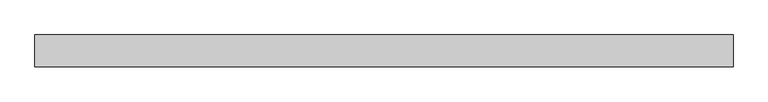
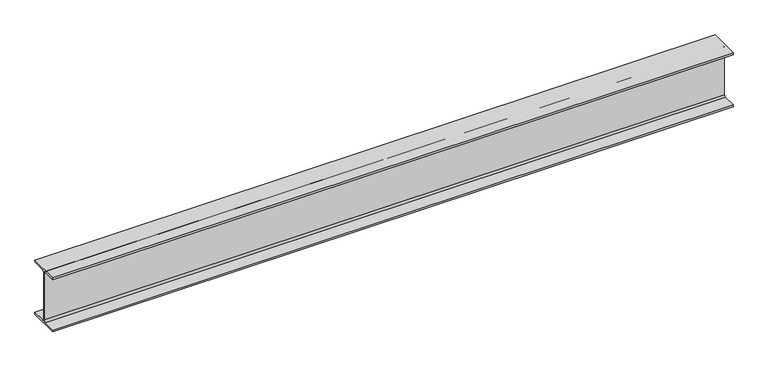
"""IFC4 building model written with IfcOpenShell, lengths in millimetres: beam geometry, Old_Steel Beam_H-KSD3502 : H_SB_ASB_H-200×200x8x12."""

from ifc_helpers import new_model, si_unit, point, frame, frame_2d, origin, place, context, project, spatial, polyline, circle_curve, trimmed, segment, composite_curve, outline, extrude, source, transform, mapped, element, save


def beam_5dc16e2d(model_context):
    return source(origin(), model_context, "Body", "SweptSolid", [
        extrude(outline(composite_curve([segment(polyline([(82.5, -141.5), (82.5, -151.7), (-82.5, -151.7), (-82.5, -141.5), (-11.9, -141.5)]), True, "CONTINUOUS"), segment(trimmed(circle_curve(frame_2d((-11.9, -132.6)), 8.9), [point((-11.9, -141.5))], [point((-3.0, -132.6))], True, "CARTESIAN"), True, "CONTINUOUS"), segment(polyline([(-3.0, -132.6), (-3.0, 132.6)]), True, "CONTINUOUS"), segment(trimmed(circle_curve(frame_2d((-11.9, 132.6)), 8.9), [point((-3.0, 132.6))], [point((-11.9, 141.5))], True, "CARTESIAN"), True, "CONTINUOUS"), segment(polyline([(-11.9, 141.5), (-82.5, 141.5), (-82.5, 151.7), (82.5, 151.7), (82.5, 141.5), (11.9, 141.5)]), True, "CONTINUOUS"), segment(trimmed(circle_curve(frame_2d((11.9, 132.6)), 8.9), [point((11.9, 141.5))], [point((3.0, 132.6))], True, "CARTESIAN"), True, "CONTINUOUS"), segment(polyline([(3.0, 132.6), (3.0, -132.6)]), True, "CONTINUOUS"), segment(trimmed(circle_curve(frame_2d((11.9, -132.6)), 8.9), [point((3.0, -132.6))], [point((11.9, -141.5))], True, "CARTESIAN"), True, "CONTINUOUS"), segment(polyline([(11.9, -141.5), (82.5, -141.5)]), True, "CONTINUOUS")], self_intersect=False)), frame((-1674.8534376, 0.0, 0.0), z_axis=(1.0, 0.0, 0.0), x_axis=(0.0, 1.0, 0.0)), (0.0, 0.0, 1.0), 3617.7011093),
    ])


if __name__ == "__main__":
    model = new_model("IFC4")
    model_context = context("Model", 3, world=origin())
    ifc_project = project(units=[si_unit("LENGTHUNIT", "METRE", prefix="MILLI")], contexts=[model_context])
    site = spatial("IfcSite", under=ifc_project)
    building = spatial("IfcBuilding", under=site)
    placement = place(None, origin())
    beam_shape = beam_5dc16e2d(model_context)
    element("IfcBeam", 1, ObjectType="Old_Steel Beam_H-KSD3502 : H_SB_ASB_H-200×200x8x12", at=placement, inside=building, context=model_context, shape_type="MappedRepresentation", body=[
        mapped(beam_shape, transform((0.0, 0.0, 0.0), x_axis=(1.0, 0.0, 0.0), y_axis=(0.0, 1.0, 0.0), z_axis=(0.0, 0.0, 1.0))),
    ])
    save(model, "model.ifc")

# Revit data of these elements
# Type "Old_Steel Beam_H-KSD3502 : H_SB_ASB_H-200×200x8x12"
#   Width = 20.0 cm
#   Web Thickness = 0.8 cm
#   Web Fillet = 1.3 cm
#   Warping Constant = 141376.0 cm⁶
#   Torsional Moment of Inertia = 26.2485 cm⁴
#   Torsional Modulus = 1.0 cm³
#   Section Area = 63.53 cm²
#   Plastic Modulus weak axis = 244.0 cm³
#   Plastic Modulus strong axis = 525.0 cm³
#   Perimeter = 1.16 m²/m
#   Nominal Weight = 49.90 kgf/m
#   Moment of Inertia weak axis = 1600.00 cm⁴
#   Moment of Inertia strong axis = 4720.00 cm⁴
#   Height = 20.0 cm
#   Flange Thickness = 1.2 cm
#   Elastic Modulus weak axis = 160.0 cm³
#   Elastic Modulus strong axis = 472.0 cm³
#   Centroid Vertical = 10.0 cm
#   Centroid Horizontal = 10.0 cm
#   Length [instance default] = 1.5240 m
#   Structural Material [instance default] = Steel, 45-345
#   Assembly Code = ""
# Element 1 (IfcBeam, "Old_Steel Beam_H-KSD3502 : H_SB_ASB_H-200×200x8x12")
#   Structural Material = none
# Materials
#   "Steel, 45-345": class "Metal", colour RGB 189 187 185, transparency 0, Description = "Steel 345 MPa", Cost = 0
